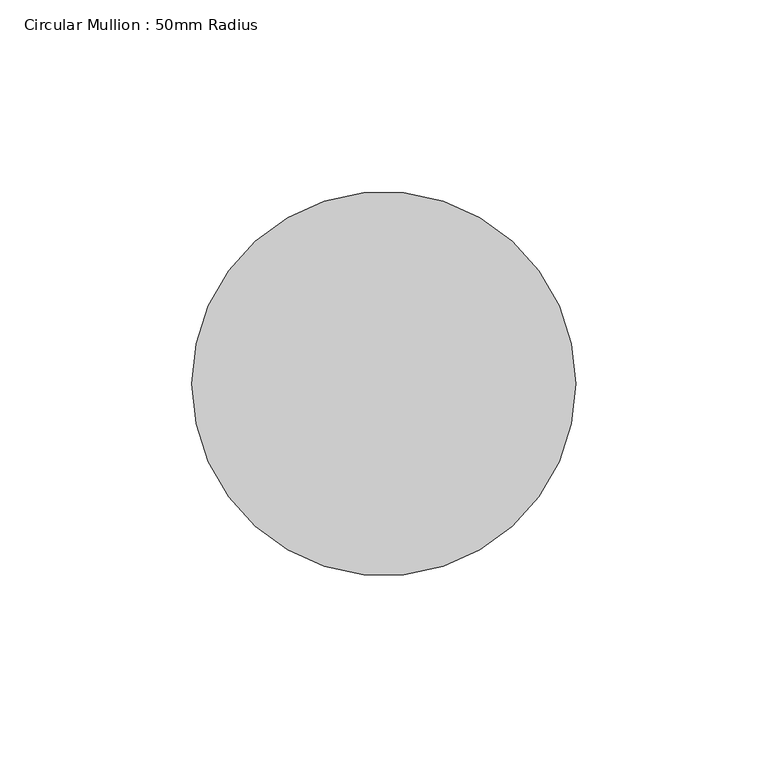
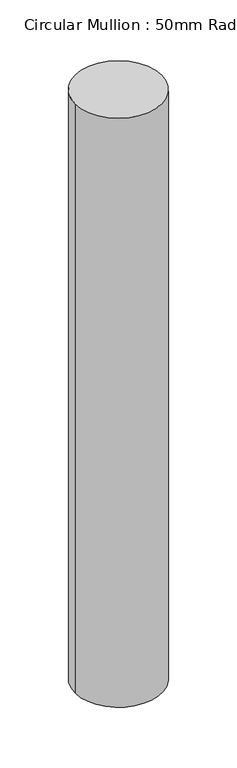
"""IFC4 building model written with IfcOpenShell, lengths in millimetres: member geometry, Circular Mullion : 50mm Radius."""

from ifc_helpers import new_model, si_unit, point, frame, origin, origin_2d, place, context, project, spatial, circle_curve, trimmed, segment, composite_curve, outline, extrude, source, transform, mapped, element, save


def circular_mullion_50mm_radius_e5f2e986(model_context):
    return source(origin(), model_context, "Body", "SweptSolid", [
        extrude(outline(composite_curve([segment(trimmed(circle_curve(origin_2d(), 50.0), [point((50.0, 0.0))], [point((-50.0, 0.0))], False, "CARTESIAN"), True, "CONTINUOUS"), segment(trimmed(circle_curve(origin_2d(), 50.0), [point((-50.0, 0.0))], [point((50.0, 0.0))], False, "CARTESIAN"), True, "CONTINUOUS")], self_intersect=False)), frame((0.0, 0.0, -717.4538951), z_axis=(0.0, 0.0, 1.0), x_axis=(1.0, 0.0, 0.0)), (0.0, 0.0, 1.0), 717.4538951),
    ])


if __name__ == "__main__":
    model = new_model("IFC4")
    model_context = context("Model", 3, world=origin())
    ifc_project = project(units=[si_unit("LENGTHUNIT", "METRE", prefix="MILLI")], contexts=[model_context])
    site = spatial("IfcSite", under=ifc_project)
    building = spatial("IfcBuilding", under=site)
    placement = place(None, origin())
    circular_mullion_50mm_radius_shape = circular_mullion_50mm_radius_e5f2e986(model_context)
    element("IfcMember", 1, ObjectType="Circular Mullion : 50mm Radius", at=placement, inside=building, context=model_context, shape_type="MappedRepresentation", body=[
        mapped(circular_mullion_50mm_radius_shape, transform((0.0, 0.0, 0.0), x_axis=(1.0, 0.0, 0.0), y_axis=(0.0, 1.0, 0.0), z_axis=(0.0, 0.0, 1.0))),
    ])
    save(model, "model.ifc")

# Revit data of these elements
# Type "Circular Mullion : 50mm Radius"
#   built-in parameter 1007350 = 0.164042 (stored number, unit not read)
# Element 1 (IfcMember, "Circular Mullion : 50mm Radius")
#   Materials on its faces: "Aluminium"
# Materials
#   "Aluminium": class "Metal", colour RGB 247 247 247, transparency 0, Description = "Aluminium 6061", Cost = 0
